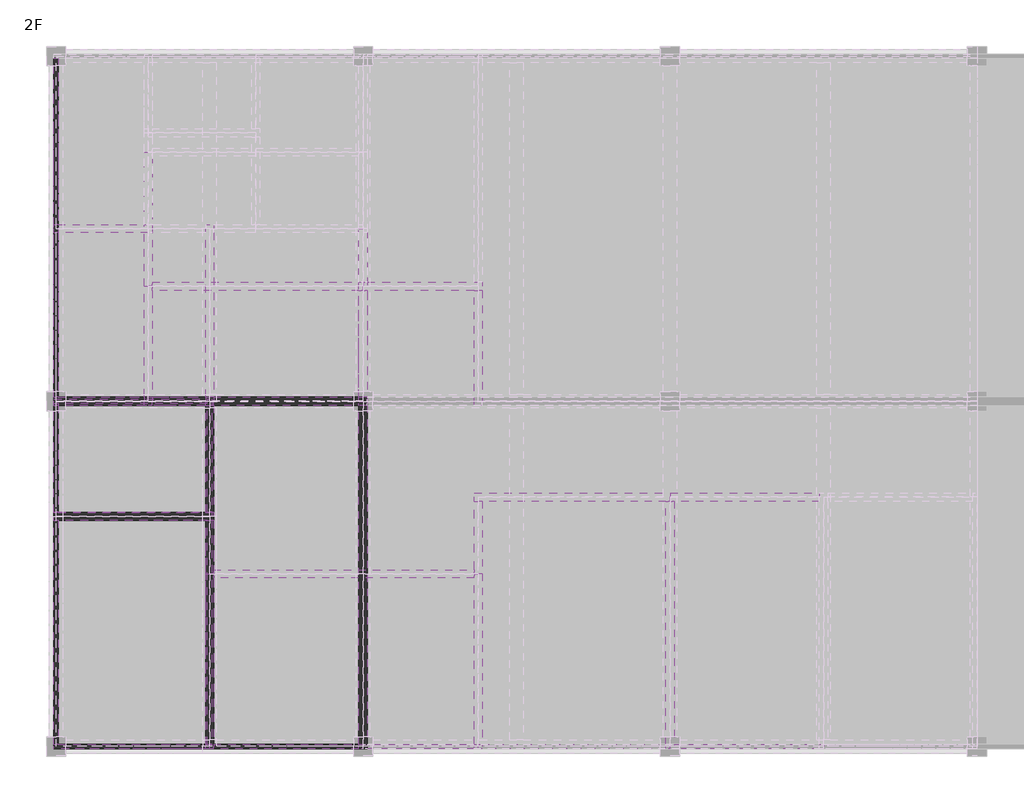
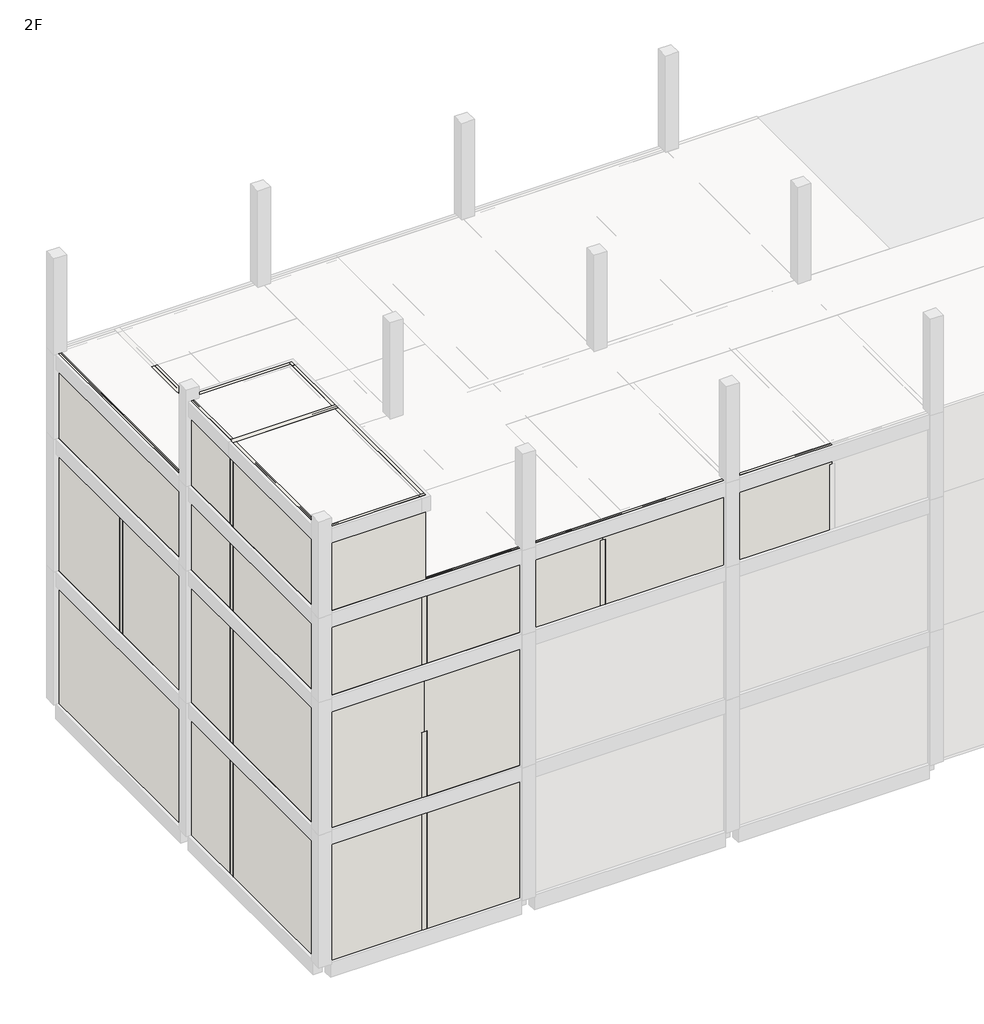
# One storey, part 1 of 7: 58 walls.
"""IFC4 building model written with IfcOpenShell, lengths in millimetres."""

from ifc_helpers import new_model, si_unit, frame, origin, place, context, project, spatial, polyline, outline, extrude, faceted_brep, element, save

model = new_model("IFC4")

# Units and contexts
model_context = context("Model", 3, world=origin())
ifc_project = project(units=[si_unit("LENGTHUNIT", "METRE", prefix="MILLI")], contexts=[model_context])

# Site, building, storey
site = spatial("IfcSite", under=ifc_project)
building = spatial("IfcBuilding", under=site)
storey = spatial("IfcBuildingStorey", under=building, Name="2F", Elevation=3500.0)

# Walls
placement = place(None, origin())
element("IfcWall", 1, ObjectType="WA211_Exterior-Cement Brick-90mm", at=placement, inside=storey, context=model_context, shape_type="SweptSolid", body=[
    extrude(outline(polyline([(45516.6521483, 181866.8614395), (45516.6521483, 173030.8614395), (45402.6521483, 173030.8614395), (45402.6521483, 181866.8614395), (45516.6521483, 181866.8614395)])), frame((0.0, 0.0, 3500.0), z_axis=(0.0, 0.0, 1.0), x_axis=(1.0, 0.0, 0.0)), (0.0, 0.0, 1.0), 5500.0),
])
element("IfcWall", 2, ObjectType="WA211_Exterior-Cement Brick-90mm", at=placement, inside=storey, context=model_context, shape_type="SweptSolid", body=[
    extrude(outline(polyline([(49566.6521483, 163980.8614395), (53352.6521483, 163980.8614395), (53352.6521483, 163866.8614395), (49566.6521483, 163866.8614395), (49566.6521483, 163980.8614395)])), frame((0.0, 0.0, 3500.0), z_axis=(0.0, 0.0, 1.0), x_axis=(1.0, 0.0, 0.0)), (0.0, 0.0, 1.0), 5500.0),
])
element("IfcWall", 3, ObjectType="WA211_Exterior-Cement Brick-90mm", at=placement, inside=storey, context=model_context, shape_type="SweptSolid", body=[
    extrude(outline(polyline([(45516.6521483, 172816.8614395), (45516.6521483, 170030.8614395), (45402.6521483, 170030.8614395), (45402.6521483, 172816.8614395), (45516.6521483, 172816.8614395)])), frame((0.0, 0.0, 3500.0), z_axis=(0.0, 0.0, 1.0), x_axis=(1.0, 0.0, 0.0)), (0.0, 0.0, 1.0), 5500.0),
])
element("IfcWall", 4, ObjectType="WA211_Exterior-Cement Brick-90mm", at=placement, inside=storey, context=model_context, shape_type="SweptSolid", body=[
    extrude(outline(polyline([(45516.6521483, 169816.8614395), (45516.6521483, 163980.8614395), (45402.6521483, 163980.8614395), (45402.6521483, 169816.8614395), (45516.6521483, 169816.8614395)])), frame((0.0, 0.0, 3500.0), z_axis=(0.0, 0.0, 1.0), x_axis=(1.0, 0.0, 0.0)), (0.0, 0.0, 1.0), 5500.0),
])
element("IfcWall", 5, ObjectType="WA211_Exterior-Cement Brick-90mm", at=placement, inside=storey, context=model_context, shape_type="Brep", body=[
    faceted_brep([(49352.6521483, 163980.8614395, 3500.0), (45516.6521483, 163980.8614395, 3500.0), (45402.6521483, 163980.8614395, 3500.0), (45402.6521483, 163980.8614395, 9000.0), (45516.6521483, 163980.8614395, 9000.0), (49352.6521483, 163980.8614395, 9000.0), (49352.6521483, 163866.8614395, 3500.0), (49352.6521483, 163866.8614395, 9000.0), (45402.6521483, 163866.8614395, 9000.0), (45402.6521483, 163866.8614395, 3500.0)], [[[0, 1, 2, 3, 4, 5]], [[6, 7, 8, 9]], [[2, 1, 0, 6, 9]], [[5, 4, 3, 8, 7]], [[0, 5, 7, 6]], [[3, 2, 9, 8]]]),
])
element("IfcWall", 6, ObjectType="WA211_Exterior-Cement Brick-90mm", at=placement, inside=storey, context=model_context, shape_type="SweptSolid", body=[
    extrude(outline(polyline([(45516.6521483, 181866.8614395), (45516.6521483, 177530.8614395), (45402.6521483, 177530.8614395), (45402.6521483, 181866.8614395), (45516.6521483, 181866.8614395)])), frame((0.0, 0.0, 9000.0), z_axis=(0.0, 0.0, 1.0), x_axis=(1.0, 0.0, 0.0)), (0.0, 0.0, 1.0), 5500.0),
])
element("IfcWall", 7, ObjectType="WA211_Exterior-Cement Brick-90mm", at=placement, inside=storey, context=model_context, shape_type="SweptSolid", body=[
    extrude(outline(polyline([(45516.6521483, 177316.8614395), (45516.6521483, 173030.8614395), (45402.6521483, 173030.8614395), (45402.6521483, 177316.8614395), (45516.6521483, 177316.8614395)])), frame((0.0, 0.0, 9000.0), z_axis=(0.0, 0.0, 1.0), x_axis=(1.0, 0.0, 0.0)), (0.0, 0.0, 1.0), 5500.0),
])
element("IfcWall", 8, ObjectType="WA211_Exterior-Cement Brick-90mm", at=placement, inside=storey, context=model_context, shape_type="SweptSolid", body=[
    extrude(outline(polyline([(45516.6521483, 172816.8614395), (45516.6521483, 170030.8614395), (45402.6521483, 170030.8614395), (45402.6521483, 172816.8614395), (45516.6521483, 172816.8614395)])), frame((0.0, 0.0, 9000.0), z_axis=(0.0, 0.0, 1.0), x_axis=(1.0, 0.0, 0.0)), (0.0, 0.0, 1.0), 5500.0),
])
element("IfcWall", 9, ObjectType="WA211_Exterior-Cement Brick-90mm", at=placement, inside=storey, context=model_context, shape_type="SweptSolid", body=[
    extrude(outline(polyline([(45516.6521483, 169816.8614395), (45516.6521483, 163980.8614395), (45402.6521483, 163980.8614395), (45402.6521483, 169816.8614395), (45516.6521483, 169816.8614395)])), frame((0.0, 0.0, 9000.0), z_axis=(0.0, 0.0, 1.0), x_axis=(1.0, 0.0, 0.0)), (0.0, 0.0, 1.0), 5500.0),
])
element("IfcWall", 10, ObjectType="WA211_Exterior-Cement Brick-90mm", at=placement, inside=storey, context=model_context, shape_type="Brep", body=[
    faceted_brep([(49352.6521483, 163980.8614395, 9000.0), (45516.6521483, 163980.8614395, 9000.0), (45402.6521483, 163980.8614395, 9000.0), (45402.6521483, 163980.8614395, 14500.0), (45516.6521483, 163980.8614395, 14500.0), (49459.6521483, 163980.8614395, 14500.0), (49459.6521483, 163980.8614395, 11700.0), (49352.6521483, 163980.8614395, 11700.0), (49352.6521483, 163866.8614395, 9000.0), (49352.6521483, 163866.8614395, 11700.0), (49459.6521483, 163866.8614395, 11700.0), (49459.6521483, 163866.8614395, 14500.0), (45402.6521483, 163866.8614395, 14500.0), (45402.6521483, 163866.8614395, 9000.0)], [[[0, 1, 2, 3, 4, 5, 6, 7]], [[8, 9, 10, 11, 12, 13]], [[2, 1, 0, 8, 13]], [[5, 4, 3, 12, 11]], [[3, 2, 13, 12]], [[6, 5, 11, 10]], [[6, 10, 9, 7]], [[0, 7, 9, 8]]]),
])
element("IfcWall", 11, ObjectType="WA211_Exterior-Cement Brick-90mm", at=placement, inside=storey, context=model_context, shape_type="SweptSolid", body=[
    extrude(outline(polyline([(9000.0, 53352.6521483), (12000.0, 53352.6521483), (12000.0, 53459.6521483), (14500.0, 53459.6521483), (14500.0, 49459.6521483), (11700.0, 49459.6521483), (11700.0, 49566.6521483), (9000.0, 49566.6521483), (9000.0, 53352.6521483)])), frame((0.0, 163866.8614395, 0.0), z_axis=(0.0, 1.0, 0.0), x_axis=(0.0, 0.0, 1.0)), (0.0, 0.0, 1.0), 114.0),
])
element("IfcWall", 12, ObjectType="WA211_Exterior-Cement Brick-90mm", at=placement, inside=storey, context=model_context, shape_type="SweptSolid", body=[
    extrude(outline(polyline([(14500.0, 65352.6521483), (17200.0, 65352.6521483), (17200.0, 65459.6521483), (18000.0, 65459.6521483), (18000.0, 61459.6521483), (17200.0, 61459.6521483), (17200.0, 61566.6521483), (14500.0, 61566.6521483), (14500.0, 65352.6521483)])), frame((0.0, 163866.8614395, 0.0), z_axis=(0.0, 1.0, 0.0), x_axis=(0.0, 0.0, 1.0)), (0.0, 0.0, 1.0), 114.0),
])
element("IfcWall", 13, ObjectType="WA211_Exterior-Cement Brick-90mm", at=placement, inside=storey, context=model_context, shape_type="SweptSolid", body=[
    extrude(outline(polyline([(14500.0, 61352.6521483), (17200.0, 61352.6521483), (17200.0, 61459.6521483), (18000.0, 61459.6521483), (18000.0, 56459.6521483), (17200.0, 56459.6521483), (17200.0, 56566.6521483), (14500.0, 56566.6521483), (14500.0, 61352.6521483)])), frame((0.0, 163866.8614395, 0.0), z_axis=(0.0, 1.0, 0.0), x_axis=(0.0, 0.0, 1.0)), (0.0, 0.0, 1.0), 114.0),
])
element("IfcWall", 14, ObjectType="WA211_Exterior-Cement Brick-90mm", at=placement, inside=storey, context=model_context, shape_type="SweptSolid", body=[
    extrude(outline(polyline([(14500.0, 56352.6521483), (17200.0, 56352.6521483), (17200.0, 56459.6521483), (18000.0, 56459.6521483), (18000.0, 49566.6521483), (14500.0, 49566.6521483), (14500.0, 56352.6521483)])), frame((0.0, 163866.8614395, 0.0), z_axis=(0.0, 1.0, 0.0), x_axis=(0.0, 0.0, 1.0)), (0.0, 0.0, 1.0), 114.0),
])
element("IfcWall", 15, ObjectType="WA211_Exterior-Cement Brick-90mm", at=placement, inside=storey, context=model_context, shape_type="SweptSolid", body=[
    extrude(outline(polyline([(45516.6521483, 181866.8614395), (45516.6521483, 173030.8614395), (45402.6521483, 173030.8614395), (45402.6521483, 181866.8614395), (45516.6521483, 181866.8614395)])), frame((0.0, 0.0, 14500.0), z_axis=(0.0, 0.0, 1.0), x_axis=(1.0, 0.0, 0.0)), (0.0, 0.0, 1.0), 3500.0),
])
element("IfcWall", 16, ObjectType="WA211_Exterior-Cement Brick-90mm", at=placement, inside=storey, context=model_context, shape_type="SweptSolid", body=[
    extrude(outline(polyline([(45516.6521483, 172816.8614395), (45516.6521483, 170030.8614395), (45402.6521483, 170030.8614395), (45402.6521483, 172816.8614395), (45516.6521483, 172816.8614395)])), frame((0.0, 0.0, 14500.0), z_axis=(0.0, 0.0, 1.0), x_axis=(1.0, 0.0, 0.0)), (0.0, 0.0, 1.0), 3500.0),
])
element("IfcWall", 17, ObjectType="WA211_Exterior-Cement Brick-90mm", at=placement, inside=storey, context=model_context, shape_type="SweptSolid", body=[
    extrude(outline(polyline([(45516.6521483, 169816.8614395), (45516.6521483, 163980.8614395), (45402.6521483, 163980.8614395), (45402.6521483, 169816.8614395), (45516.6521483, 169816.8614395)])), frame((0.0, 0.0, 14500.0), z_axis=(0.0, 0.0, 1.0), x_axis=(1.0, 0.0, 0.0)), (0.0, 0.0, 1.0), 3500.0),
])
element("IfcWall", 18, ObjectType="WA211_Exterior-Cement Brick-90mm", at=placement, inside=storey, context=model_context, shape_type="Brep", body=[
    faceted_brep([(49352.6521483, 163980.8614395, 14500.0), (45516.6521483, 163980.8614395, 14500.0), (45402.6521483, 163980.8614395, 14500.0), (45402.6521483, 163980.8614395, 18000.0), (45516.6521483, 163980.8614395, 18000.0), (49352.6521483, 163980.8614395, 18000.0), (49352.6521483, 163866.8614395, 14500.0), (49352.6521483, 163866.8614395, 18000.0), (45402.6521483, 163866.8614395, 18000.0), (45402.6521483, 163866.8614395, 14500.0)], [[[0, 1, 2, 3, 4, 5]], [[6, 7, 8, 9]], [[2, 1, 0, 6, 9]], [[5, 4, 3, 8, 7]], [[0, 5, 7, 6]], [[3, 2, 9, 8]]]),
])
element("IfcWall", 19, ObjectType="WA211_Exterior-Cement Brick-90mm", at=placement, inside=storey, context=model_context, shape_type="Brep", body=[
    faceted_brep([(49402.6521483, 172980.8614395, 18000.0), (49402.6521483, 172866.8614395, 18000.0), (49402.6521483, 170030.8614395, 18000.0), (49402.6521483, 170030.8614395, 21500.0), (49402.6521483, 172866.8614395, 21500.0), (49402.6521483, 172980.8614395, 21500.0), (49516.6521483, 172980.8614395, 18000.0), (49516.6521483, 172980.8614395, 21500.0), (49516.6521483, 170030.8614395, 21500.0), (49516.6521483, 170030.8614395, 18000.0)], [[[0, 1, 2, 3, 4, 5]], [[6, 7, 8, 9]], [[2, 1, 0, 6, 9]], [[5, 4, 3, 8, 7]], [[0, 5, 7, 6]], [[3, 2, 9, 8]]]),
])
element("IfcWall", 20, ObjectType="WA211_Exterior-Cement Brick-90mm", at=placement, inside=storey, context=model_context, shape_type="SweptSolid", body=[
    extrude(outline(polyline([(45516.6521483, 172866.8614395), (45516.6521483, 170030.8614395), (45402.6521483, 170030.8614395), (45402.6521483, 172866.8614395), (45516.6521483, 172866.8614395)])), frame((0.0, 0.0, 18000.0), z_axis=(0.0, 0.0, 1.0), x_axis=(1.0, 0.0, 0.0)), (0.0, 0.0, 1.0), 3500.0),
])
element("IfcWall", 21, ObjectType="WA211_Exterior-Cement Brick-90mm", at=placement, inside=storey, context=model_context, shape_type="Brep", body=[
    faceted_brep([(45402.6521483, 172866.8614395, 18000.0), (45516.6521483, 172866.8614395, 18000.0), (49402.6521483, 172866.8614395, 18000.0), (49402.6521483, 172866.8614395, 21500.0), (45516.6521483, 172866.8614395, 21500.0), (45402.6521483, 172866.8614395, 21500.0), (45402.6521483, 172980.8614395, 18000.0), (45402.6521483, 172980.8614395, 21500.0), (49402.6521483, 172980.8614395, 21500.0), (49402.6521483, 172980.8614395, 18000.0)], [[[0, 1, 2, 3, 4, 5]], [[6, 7, 8, 9]], [[2, 1, 0, 6, 9]], [[5, 4, 3, 8, 7]], [[0, 5, 7, 6]], [[3, 2, 9, 8]]]),
])
element("IfcWall", 22, ObjectType="WA211_Exterior-Cement Brick-90mm", at=placement, inside=storey, context=model_context, shape_type="SweptSolid", body=[
    extrude(outline(polyline([(45516.6521483, 169816.8614395), (45516.6521483, 163980.8614395), (45402.6521483, 163980.8614395), (45402.6521483, 169816.8614395), (45516.6521483, 169816.8614395)])), frame((0.0, 0.0, 18000.0), z_axis=(0.0, 0.0, 1.0), x_axis=(1.0, 0.0, 0.0)), (0.0, 0.0, 1.0), 3500.0),
])
element("IfcWall", 23, ObjectType="WA211_Exterior-Cement Brick-90mm", at=placement, inside=storey, context=model_context, shape_type="Brep", body=[
    faceted_brep([(49516.6521483, 163980.8614395, 18000.0), (49402.6521483, 163980.8614395, 18000.0), (45516.6521483, 163980.8614395, 18000.0), (45402.6521483, 163980.8614395, 18000.0), (45402.6521483, 163980.8614395, 21500.0), (45516.6521483, 163980.8614395, 21500.0), (49402.6521483, 163980.8614395, 21500.0), (49516.6521483, 163980.8614395, 21500.0), (49516.6521483, 163866.8614395, 18000.0), (49516.6521483, 163866.8614395, 21500.0), (45402.6521483, 163866.8614395, 21500.0), (45402.6521483, 163866.8614395, 18000.0)], [[[0, 1, 2, 3, 4, 5, 6, 7]], [[8, 9, 10, 11]], [[3, 2, 1, 0, 8, 11]], [[7, 6, 5, 4, 10, 9]], [[0, 7, 9, 8]], [[4, 3, 11, 10]]]),
])
element("IfcWall", 24, ObjectType="WA211_Exterior-Cement Brick-90mm", at=placement, inside=storey, context=model_context, shape_type="SweptSolid", body=[
    extrude(outline(polyline([(49402.6521483, 163980.8614395), (49402.6521483, 169816.8614395), (49516.6521483, 169816.8614395), (49516.6521483, 163980.8614395), (49402.6521483, 163980.8614395)])), frame((0.0, 0.0, 18000.0), z_axis=(0.0, 0.0, 1.0), x_axis=(1.0, 0.0, 0.0)), (0.0, 0.0, 1.0), 3500.0),
])
element("IfcWall", 25, ObjectType="WA221_Interior-Cement Block-190mm", at=placement, inside=storey, context=model_context, shape_type="SweptSolid", body=[
    extrude(outline(polyline([(49566.6521483, 173030.8614395), (53352.6521483, 173030.8614395), (53352.6521483, 172816.8614395), (49566.6521483, 172816.8614395), (49566.6521483, 173030.8614395)])), frame((0.0, 0.0, 3500.0), z_axis=(0.0, 0.0, 1.0), x_axis=(1.0, 0.0, 0.0)), (0.0, 0.0, 1.0), 5500.0),
])
element("IfcWall", 26, ObjectType="WA221_Interior-Cement Block-190mm", at=placement, inside=storey, context=model_context, shape_type="Brep", body=[
    faceted_brep([(45402.6521483, 172816.8614395, 3500.0), (45516.6521483, 172816.8614395, 3500.0), (49352.6521483, 172816.8614395, 3500.0), (49352.6521483, 172816.8614395, 9000.0), (45516.6521483, 172816.8614395, 9000.0), (45402.6521483, 172816.8614395, 9000.0), (45402.6521483, 173030.8614395, 3500.0), (45402.6521483, 173030.8614395, 9000.0), (45516.6521483, 173030.8614395, 9000.0), (49352.6521483, 173030.8614395, 9000.0), (49352.6521483, 173030.8614395, 3500.0), (45516.6521483, 173030.8614395, 3500.0)], [[[0, 1, 2, 3, 4, 5]], [[6, 7, 8, 9, 10, 11]], [[2, 1, 0, 6, 11, 10]], [[5, 4, 3, 9, 8, 7]], [[0, 5, 7, 6]], [[3, 2, 10, 9]]]),
])
element("IfcWall", 27, ObjectType="WA221_Interior-Cement Block-190mm", at=placement, inside=storey, context=model_context, shape_type="Brep", body=[
    faceted_brep([(53566.6521483, 163866.8614395, 3500.0), (53566.6521483, 163980.8614395, 3500.0), (53566.6521483, 172816.8614395, 3500.0), (53566.6521483, 173030.8614395, 3500.0), (53566.6521483, 173030.8614395, 9000.0), (53566.6521483, 172816.8614395, 9000.0), (53566.6521483, 163980.8614395, 9000.0), (53566.6521483, 163866.8614395, 9000.0), (53352.6521483, 163866.8614395, 3500.0), (53352.6521483, 163866.8614395, 9000.0), (53352.6521483, 163980.8614395, 9000.0), (53352.6521483, 172816.8614395, 9000.0), (53352.6521483, 173030.8614395, 9000.0), (53352.6521483, 173030.8614395, 3500.0), (53352.6521483, 172816.8614395, 3500.0), (53352.6521483, 163980.8614395, 3500.0)], [[[0, 1, 2, 3, 4, 5, 6, 7]], [[8, 9, 10, 11, 12, 13, 14, 15]], [[3, 2, 1, 0, 8, 15, 14, 13]], [[7, 6, 5, 4, 12, 11, 10, 9]], [[0, 7, 9, 8]], [[4, 3, 13, 12]]]),
])
element("IfcWall", 28, ObjectType="WA221_Interior-Cement Block-190mm", at=placement, inside=storey, context=model_context, shape_type="Brep", body=[
    faceted_brep([(49352.6521483, 173030.8614395, 3500.0), (49352.6521483, 172816.8614395, 3500.0), (49352.6521483, 170030.8614395, 3500.0), (49352.6521483, 170030.8614395, 9000.0), (49352.6521483, 172816.8614395, 9000.0), (49352.6521483, 173030.8614395, 9000.0), (49566.6521483, 173030.8614395, 3500.0), (49566.6521483, 173030.8614395, 9000.0), (49566.6521483, 172816.8614395, 9000.0), (49566.6521483, 170030.8614395, 9000.0), (49566.6521483, 170030.8614395, 3500.0), (49566.6521483, 172816.8614395, 3500.0)], [[[0, 1, 2, 3, 4, 5]], [[6, 7, 8, 9, 10, 11]], [[2, 1, 0, 6, 11, 10]], [[5, 4, 3, 9, 8, 7]], [[0, 5, 7, 6]], [[3, 2, 10, 9]]]),
])
element("IfcWall", 29, ObjectType="WA221_Interior-Cement Block-190mm", at=placement, inside=storey, context=model_context, shape_type="Brep", body=[
    faceted_brep([(49352.6521483, 169816.8614395, 3500.0), (49352.6521483, 163980.8614395, 3500.0), (49352.6521483, 163866.8614395, 3500.0), (49352.6521483, 163866.8614395, 9000.0), (49352.6521483, 163980.8614395, 9000.0), (49352.6521483, 169816.8614395, 9000.0), (49566.6521483, 169816.8614395, 3500.0), (49566.6521483, 169816.8614395, 9000.0), (49566.6521483, 163980.8614395, 9000.0), (49566.6521483, 163866.8614395, 9000.0), (49566.6521483, 163866.8614395, 3500.0), (49566.6521483, 163980.8614395, 3500.0)], [[[0, 1, 2, 3, 4, 5]], [[6, 7, 8, 9, 10, 11]], [[2, 1, 0, 6, 11, 10]], [[5, 4, 3, 9, 8, 7]], [[3, 2, 10, 9]], [[0, 5, 7, 6]]]),
])
element("IfcWall", 30, ObjectType="WA221_Interior-Cement Block-190mm", at=placement, inside=storey, context=model_context, shape_type="Brep", body=[
    faceted_brep([(45402.6521483, 169816.8614395, 3500.0), (45516.6521483, 169816.8614395, 3500.0), (49352.6521483, 169816.8614395, 3500.0), (49566.6521483, 169816.8614395, 3500.0), (49566.6521483, 169816.8614395, 9000.0), (49352.6521483, 169816.8614395, 9000.0), (45516.6521483, 169816.8614395, 9000.0), (45402.6521483, 169816.8614395, 9000.0), (45402.6521483, 170030.8614395, 3500.0), (45402.6521483, 170030.8614395, 9000.0), (45516.6521483, 170030.8614395, 9000.0), (49352.6521483, 170030.8614395, 9000.0), (49566.6521483, 170030.8614395, 9000.0), (49566.6521483, 170030.8614395, 3500.0), (49352.6521483, 170030.8614395, 3500.0), (45516.6521483, 170030.8614395, 3500.0)], [[[0, 1, 2, 3, 4, 5, 6, 7]], [[8, 9, 10, 11, 12, 13, 14, 15]], [[3, 2, 1, 0, 8, 15, 14, 13]], [[7, 6, 5, 4, 12, 11, 10, 9]], [[0, 7, 9, 8]], [[4, 3, 13, 12]]]),
])
element("IfcWall", 31, ObjectType="WA221_Interior-Cement Block-190mm", at=placement, inside=storey, context=model_context, shape_type="Brep", body=[
    faceted_brep([(53566.6521483, 172923.8614395, 9000.0), (53566.6521483, 173030.8614395, 9000.0), (53566.6521483, 177316.8614395, 9000.0), (53566.6521483, 177316.8614395, 11700.0), (53566.6521483, 177423.8614395, 11700.0), (53566.6521483, 177423.8614395, 12400.0), (53566.6521483, 173030.8614395, 12400.0), (53566.6521483, 172816.8614395, 12400.0), (53566.6521483, 172816.8614395, 12000.0), (53566.6521483, 172923.8614395, 12000.0), (53352.6521483, 172923.8614395, 9000.0), (53352.6521483, 172923.8614395, 12000.0), (53352.6521483, 172816.8614395, 12000.0), (53352.6521483, 172816.8614395, 12400.0), (53352.6521483, 177423.8614395, 12400.0), (53352.6521483, 177423.8614395, 11700.0), (53352.6521483, 177316.8614395, 11700.0), (53352.6521483, 177316.8614395, 9000.0)], [[[0, 1, 2, 3, 4, 5, 6, 7, 8, 9]], [[10, 11, 12, 13, 14, 15, 16, 17]], [[2, 1, 0, 10, 17]], [[7, 6, 5, 14, 13]], [[0, 9, 11, 10]], [[8, 12, 11, 9]], [[8, 7, 13, 12]], [[5, 4, 15, 14]], [[15, 4, 3, 16]], [[3, 2, 17, 16]]]),
])
element("IfcWall", 32, ObjectType="WA221_Interior-Cement Block-190mm", at=placement, inside=storey, context=model_context, shape_type="Brep", body=[
    faceted_brep([(53566.6521483, 163866.8614395, 9000.0), (53566.6521483, 163980.8614395, 9000.0), (53566.6521483, 172816.8614395, 9000.0), (53566.6521483, 172923.8614395, 9000.0), (53566.6521483, 172923.8614395, 12000.0), (53566.6521483, 172816.8614395, 12000.0), (53566.6521483, 163980.8614395, 12000.0), (53566.6521483, 163866.8614395, 12000.0), (53352.6521483, 163866.8614395, 9000.0), (53352.6521483, 163866.8614395, 12000.0), (53352.6521483, 163980.8614395, 12000.0), (53352.6521483, 172816.8614395, 12000.0), (53352.6521483, 172923.8614395, 12000.0), (53352.6521483, 172923.8614395, 9000.0), (53352.6521483, 163980.8614395, 9000.0), (53459.6521483, 163866.8614395, 12000.0)], [[[0, 1, 2, 3, 4, 5, 6, 7]], [[8, 9, 10, 11, 12, 13, 14]], [[3, 2, 1, 0, 8, 14, 13]], [[4, 3, 13, 12]], [[7, 6, 5, 4, 12, 11, 10, 9, 15]], [[0, 7, 15, 9, 8]]]),
])
element("IfcWall", 33, ObjectType="WA221_Interior-Cement Block-190mm", at=placement, inside=storey, context=model_context, shape_type="Brep", body=[
    faceted_brep([(47859.6521483, 177530.8614395, 9000.0), (47752.6521483, 177530.8614395, 9000.0), (45516.6521483, 177530.8614395, 9000.0), (45402.6521483, 177530.8614395, 9000.0), (45402.6521483, 177530.8614395, 14500.0), (45516.6521483, 177530.8614395, 14500.0), (47752.6521483, 177530.8614395, 14500.0), (47966.6521483, 177530.8614395, 14500.0), (47966.6521483, 177530.8614395, 11700.0), (47859.6521483, 177530.8614395, 11700.0), (47859.6521483, 177316.8614395, 9000.0), (47859.6521483, 177316.8614395, 11700.0), (47966.6521483, 177316.8614395, 11700.0), (47966.6521483, 177316.8614395, 14500.0), (45516.6521483, 177316.8614395, 14500.0), (45402.6521483, 177316.8614395, 14500.0), (45402.6521483, 177316.8614395, 9000.0), (45516.6521483, 177316.8614395, 9000.0)], [[[0, 1, 2, 3, 4, 5, 6, 7, 8, 9]], [[10, 11, 12, 13, 14, 15, 16, 17]], [[3, 2, 1, 0, 10, 17, 16]], [[7, 6, 5, 4, 15, 14, 13]], [[0, 9, 11, 10]], [[8, 12, 11, 9]], [[8, 7, 13, 12]], [[4, 3, 16, 15]]]),
])
element("IfcWall", 34, ObjectType="WA221_Interior-Cement Block-190mm", at=placement, inside=storey, context=model_context, shape_type="Brep", body=[
    faceted_brep([(45402.6521483, 172816.8614395, 9000.0), (45516.6521483, 172816.8614395, 9000.0), (49352.6521483, 172816.8614395, 9000.0), (49566.6521483, 172816.8614395, 9000.0), (49566.6521483, 172816.8614395, 14500.0), (49352.6521483, 172816.8614395, 14500.0), (45516.6521483, 172816.8614395, 14500.0), (45402.6521483, 172816.8614395, 14500.0), (45402.6521483, 173030.8614395, 9000.0), (45402.6521483, 173030.8614395, 14500.0), (45516.6521483, 173030.8614395, 14500.0), (49566.6521483, 173030.8614395, 14500.0), (49566.6521483, 173030.8614395, 11700.0), (49566.6521483, 173030.8614395, 9000.0), (49352.6521483, 173030.8614395, 9000.0), (45516.6521483, 173030.8614395, 9000.0)], [[[0, 1, 2, 3, 4, 5, 6, 7]], [[8, 9, 10, 11, 12, 13, 14, 15]], [[3, 2, 1, 0, 8, 15, 14, 13]], [[7, 6, 5, 4, 11, 10, 9]], [[0, 7, 9, 8]], [[3, 13, 12, 11, 4]]]),
])
element("IfcWall", 35, ObjectType="WA221_Interior-Cement Block-190mm", at=placement, inside=storey, context=model_context, shape_type="Brep", body=[
    faceted_brep([(49352.6521483, 177530.8614395, 9000.0), (49352.6521483, 177316.8614395, 9000.0), (49352.6521483, 173030.8614395, 9000.0), (49352.6521483, 173030.8614395, 11700.0), (49352.6521483, 177316.8614395, 11700.0), (49352.6521483, 177530.8614395, 11700.0), (49566.6521483, 177530.8614395, 9000.0), (49566.6521483, 177530.8614395, 11700.0), (49566.6521483, 177316.8614395, 11700.0), (49566.6521483, 173030.8614395, 11700.0), (49566.6521483, 173030.8614395, 9000.0), (49566.6521483, 177316.8614395, 9000.0)], [[[0, 1, 2, 3, 4, 5]], [[6, 7, 8, 9, 10, 11]], [[2, 1, 0, 6, 11, 10]], [[5, 4, 3, 9, 8, 7]], [[0, 5, 7, 6]], [[3, 2, 10, 9]]]),
])
element("IfcWall", 36, ObjectType="WA221_Interior-Cement Block-190mm", at=placement, inside=storey, context=model_context, shape_type="Brep", body=[
    faceted_brep([(49566.6521483, 170030.8614395, 14500.0), (49566.6521483, 170030.8614395, 9000.0), (49352.6521483, 170030.8614395, 9000.0), (45516.6521483, 170030.8614395, 9000.0), (45402.6521483, 170030.8614395, 9000.0), (45402.6521483, 170030.8614395, 14500.0), (45516.6521483, 170030.8614395, 14500.0), (49352.6521483, 170030.8614395, 14500.0), (49566.6521483, 169816.8614395, 9000.0), (49566.6521483, 169816.8614395, 11700.0), (49566.6521483, 169816.8614395, 14500.0), (45516.6521483, 169816.8614395, 14500.0), (45402.6521483, 169816.8614395, 14500.0), (45402.6521483, 169816.8614395, 9000.0), (45516.6521483, 169816.8614395, 9000.0), (49352.6521483, 169816.8614395, 9000.0)], [[[0, 1, 2, 3, 4, 5, 6, 7]], [[8, 9, 10, 11, 12, 13, 14, 15]], [[4, 3, 2, 1, 8, 15, 14, 13]], [[0, 7, 6, 5, 12, 11, 10]], [[5, 4, 13, 12]], [[0, 10, 9, 8, 1]]]),
])
element("IfcWall", 37, ObjectType="WA221_Interior-Cement Block-190mm", at=placement, inside=storey, context=model_context, shape_type="SweptSolid", body=[
    extrude(outline(polyline([(49352.6521483, 170030.8614395), (49352.6521483, 172816.8614395), (49566.6521483, 172816.8614395), (49566.6521483, 170030.8614395), (49352.6521483, 170030.8614395)])), frame((0.0, 0.0, 9000.0), z_axis=(0.0, 0.0, 1.0), x_axis=(1.0, 0.0, 0.0)), (0.0, 0.0, 1.0), 5500.0),
])
element("IfcWall", 38, ObjectType="WA221_Interior-Cement Block-190mm", at=placement, inside=storey, context=model_context, shape_type="Brep", body=[
    faceted_brep([(49352.6521483, 169816.8614395, 9000.0), (49352.6521483, 163980.8614395, 9000.0), (49352.6521483, 163866.8614395, 9000.0), (49352.6521483, 163866.8614395, 11700.0), (49352.6521483, 163980.8614395, 11700.0), (49352.6521483, 169816.8614395, 11700.0), (49566.6521483, 169816.8614395, 9000.0), (49566.6521483, 169816.8614395, 11700.0), (49566.6521483, 163980.8614395, 11700.0), (49566.6521483, 163866.8614395, 11700.0), (49566.6521483, 163866.8614395, 9000.0), (49566.6521483, 163980.8614395, 9000.0), (49459.6521483, 163866.8614395, 11700.0)], [[[0, 1, 2, 3, 4, 5]], [[6, 7, 8, 9, 10, 11]], [[2, 1, 0, 6, 11, 10]], [[5, 4, 3, 12, 9, 8, 7]], [[0, 5, 7, 6]], [[3, 2, 10, 9, 12]]]),
])
element("IfcWall", 39, ObjectType="WA221_Interior-Cement Block-190mm", at=placement, inside=storey, context=model_context, shape_type="Brep", body=[
    faceted_brep([(61352.6521483, 170316.8614395, 14500.0), (61352.6521483, 163980.8614395, 14500.0), (61352.6521483, 163866.8614395, 14500.0), (61352.6521483, 163866.8614395, 17200.0), (61352.6521483, 163980.8614395, 17200.0), (61352.6521483, 170316.8614395, 17200.0), (61566.6521483, 170316.8614395, 14500.0), (61566.6521483, 170316.8614395, 17200.0), (61566.6521483, 163980.8614395, 17200.0), (61566.6521483, 163866.8614395, 17200.0), (61566.6521483, 163866.8614395, 14500.0), (61566.6521483, 163980.8614395, 14500.0), (61459.6521483, 170316.8614395, 14500.0), (61459.6521483, 163866.8614395, 17200.0), (61459.6521483, 170316.8614395, 17200.0)], [[[0, 1, 2, 3, 4, 5]], [[6, 7, 8, 9, 10, 11]], [[2, 1, 0, 12, 6, 11, 10]], [[5, 4, 3, 13, 9, 8, 7, 14]], [[3, 2, 10, 9, 13]], [[0, 5, 14, 7, 6, 12]]]),
])
element("IfcWall", 40, ObjectType="WA221_Interior-Cement Block-190mm", at=placement, inside=storey, context=model_context, shape_type="Brep", body=[
    faceted_brep([(61459.6521483, 170316.8614395, 14500.0), (61566.6521483, 170316.8614395, 14500.0), (65352.6521483, 170316.8614395, 14500.0), (65352.6521483, 170316.8614395, 17200.0), (61566.6521483, 170316.8614395, 17200.0), (61459.6521483, 170316.8614395, 17200.0), (61459.6521483, 170530.8614395, 14500.0), (61459.6521483, 170530.8614395, 17200.0), (65352.6521483, 170530.8614395, 17200.0), (65352.6521483, 170530.8614395, 14500.0)], [[[0, 1, 2, 3, 4, 5]], [[6, 7, 8, 9]], [[2, 1, 0, 6, 9]], [[5, 4, 3, 8, 7]], [[0, 5, 7, 6]], [[3, 2, 9, 8]]]),
])
element("IfcWall", 41, ObjectType="WA221_Interior-Cement Block-190mm", at=placement, inside=storey, context=model_context, shape_type="Brep", body=[
    faceted_brep([(56566.6521483, 172816.8614395, 14500.0), (56566.6521483, 173030.8614395, 14500.0), (56566.6521483, 175816.8614395, 14500.0), (56566.6521483, 175816.8614395, 17200.0), (56566.6521483, 173030.8614395, 17200.0), (56566.6521483, 172816.8614395, 17200.0), (56352.6521483, 172816.8614395, 14500.0), (56352.6521483, 172816.8614395, 17200.0), (56352.6521483, 175816.8614395, 17200.0), (56352.6521483, 175816.8614395, 14500.0)], [[[0, 1, 2, 3, 4, 5]], [[6, 7, 8, 9]], [[2, 1, 0, 6, 9]], [[5, 4, 3, 8, 7]], [[0, 5, 7, 6]], [[3, 2, 9, 8]]]),
])
element("IfcWall", 42, ObjectType="WA221_Interior-Cement Block-190mm", at=placement, inside=storey, context=model_context, shape_type="Brep", body=[
    faceted_brep([(56566.6521483, 163866.8614395, 14500.0), (56566.6521483, 163980.8614395, 14500.0), (56566.6521483, 168423.8614395, 14500.0), (56566.6521483, 168423.8614395, 17200.0), (56566.6521483, 163980.8614395, 17200.0), (56566.6521483, 163866.8614395, 17200.0), (56352.6521483, 163866.8614395, 14500.0), (56352.6521483, 163866.8614395, 17200.0), (56352.6521483, 163980.8614395, 17200.0), (56352.6521483, 168316.8614395, 17200.0), (56352.6521483, 168423.8614395, 17200.0), (56352.6521483, 168423.8614395, 14500.0), (56352.6521483, 168316.8614395, 14500.0), (56352.6521483, 163980.8614395, 14500.0), (56459.6521483, 163866.8614395, 17200.0)], [[[0, 1, 2, 3, 4, 5]], [[6, 7, 8, 9, 10, 11, 12, 13]], [[2, 1, 0, 6, 13, 12, 11]], [[3, 2, 11, 10]], [[5, 4, 3, 10, 9, 8, 7, 14]], [[0, 5, 14, 7, 6]]]),
])
element("IfcWall", 43, ObjectType="WA221_Interior-Cement Block-190mm", at=placement, inside=storey, context=model_context, shape_type="Brep", body=[
    faceted_brep([(56352.6521483, 170316.8614395, 14500.0), (56566.6521483, 170316.8614395, 14500.0), (61352.6521483, 170316.8614395, 14500.0), (61459.6521483, 170316.8614395, 14500.0), (61459.6521483, 170316.8614395, 17200.0), (61352.6521483, 170316.8614395, 17200.0), (56566.6521483, 170316.8614395, 17200.0), (56352.6521483, 170316.8614395, 17200.0), (56352.6521483, 170530.8614395, 14500.0), (56352.6521483, 170530.8614395, 17200.0), (61459.6521483, 170530.8614395, 17200.0), (61459.6521483, 170530.8614395, 14500.0)], [[[0, 1, 2, 3, 4, 5, 6, 7]], [[8, 9, 10, 11]], [[3, 2, 1, 0, 8, 11]], [[4, 3, 11, 10]], [[7, 6, 5, 4, 10, 9]], [[0, 7, 9, 8]]]),
])
element("IfcWall", 44, ObjectType="WA221_Interior-Cement Block-190mm", at=placement, inside=storey, context=model_context, shape_type="Brep", body=[
    faceted_brep([(56566.6521483, 168423.8614395, 14500.0), (56566.6521483, 170316.8614395, 14500.0), (56566.6521483, 170316.8614395, 17200.0), (56566.6521483, 168423.8614395, 17200.0), (56352.6521483, 168423.8614395, 14500.0), (56352.6521483, 168423.8614395, 17200.0), (56352.6521483, 168530.8614395, 17200.0), (56352.6521483, 170316.8614395, 17200.0), (56352.6521483, 170316.8614395, 14500.0), (56352.6521483, 168530.8614395, 14500.0)], [[[0, 1, 2, 3]], [[4, 5, 6, 7, 8, 9]], [[1, 0, 4, 9, 8]], [[3, 2, 7, 6, 5]], [[0, 3, 5, 4]], [[2, 1, 8, 7]]]),
])
element("IfcWall", 45, ObjectType="WA221_Interior-Cement Block-190mm", at=placement, inside=storey, context=model_context, shape_type="Brep", body=[
    faceted_brep([(49352.6521483, 168423.8614395, 18000.0), (49352.6521483, 168423.8614395, 14500.0), (49352.6521483, 163980.8614395, 14500.0), (49352.6521483, 163866.8614395, 14500.0), (49352.6521483, 163866.8614395, 18000.0), (49352.6521483, 163980.8614395, 18000.0), (49566.6521483, 168423.8614395, 14500.0), (49566.6521483, 168423.8614395, 18000.0), (49566.6521483, 163980.8614395, 18000.0), (49566.6521483, 163866.8614395, 18000.0), (49566.6521483, 163866.8614395, 14500.0), (49566.6521483, 163980.8614395, 14500.0), (49566.6521483, 168316.8614395, 14500.0)], [[[0, 1, 2, 3, 4, 5]], [[6, 7, 8, 9, 10, 11, 12]], [[3, 2, 1, 6, 12, 11, 10]], [[0, 5, 4, 9, 8, 7]], [[0, 7, 6, 1]], [[4, 3, 10, 9]]]),
])
element("IfcWall", 46, ObjectType="WA221_Interior-Cement Block-190mm", at=placement, inside=storey, context=model_context, shape_type="Brep", body=[
    faceted_brep([(56352.6521483, 168530.8614395, 14500.0), (49566.6521483, 168530.8614395, 14500.0), (49566.6521483, 168530.8614395, 17200.0), (56352.6521483, 168530.8614395, 17200.0), (56352.6521483, 168316.8614395, 14500.0), (56352.6521483, 168316.8614395, 17200.0), (49566.6521483, 168316.8614395, 17200.0), (49566.6521483, 168316.8614395, 14500.0), (56352.6521483, 168423.8614395, 14500.0), (49566.6521483, 168423.8614395, 14500.0), (56352.6521483, 168423.8614395, 17200.0)], [[[0, 1, 2, 3]], [[4, 5, 6, 7]], [[1, 0, 8, 4, 7, 9]], [[3, 2, 6, 5, 10]], [[0, 3, 10, 5, 4, 8]], [[2, 1, 9, 7, 6]]]),
])
element("IfcWall", 47, ObjectType="WA221_Interior-Cement Block-190mm", at=placement, inside=storey, context=model_context, shape_type="Brep", body=[
    faceted_brep([(47966.6521483, 175816.8614395, 14500.0), (53352.6521483, 175816.8614395, 14500.0), (53459.6521483, 175816.8614395, 14500.0), (53459.6521483, 175816.8614395, 17200.0), (53352.6521483, 175816.8614395, 17200.0), (47966.6521483, 175816.8614395, 17200.0), (47966.6521483, 176030.8614395, 14500.0), (47966.6521483, 176030.8614395, 17200.0), (53352.6521483, 176030.8614395, 17200.0), (53459.6521483, 176030.8614395, 17200.0), (53459.6521483, 176030.8614395, 14500.0), (53352.6521483, 176030.8614395, 14500.0), (47966.6521483, 175923.8614395, 14500.0)], [[[0, 1, 2, 3, 4, 5]], [[6, 7, 8, 9, 10, 11]], [[2, 1, 0, 12, 6, 11, 10]], [[3, 2, 10, 9]], [[5, 4, 3, 9, 8, 7]], [[0, 5, 7, 6, 12]]]),
])
element("IfcWall", 48, ObjectType="WA221_Interior-Cement Block-190mm", at=placement, inside=storey, context=model_context, shape_type="Brep", body=[
    faceted_brep([(47752.6521483, 179423.8614395, 18000.0), (47752.6521483, 179423.8614395, 14500.0), (47752.6521483, 175923.8614395, 14500.0), (47752.6521483, 175923.8614395, 18000.0), (47966.6521483, 179423.8614395, 14500.0), (47966.6521483, 179423.8614395, 18000.0), (47966.6521483, 175923.8614395, 18000.0), (47966.6521483, 175923.8614395, 14500.0), (47966.6521483, 176030.8614395, 14500.0), (47966.6521483, 179316.8614395, 14500.0)], [[[0, 1, 2, 3]], [[4, 5, 6, 7, 8, 9]], [[2, 1, 4, 9, 8, 7]], [[0, 3, 6, 5]], [[0, 5, 4, 1]], [[2, 7, 6, 3]]]),
])
element("IfcWall", 49, ObjectType="WA221_Interior-Cement Block-190mm", at=placement, inside=storey, context=model_context, shape_type="Brep", body=[
    faceted_brep([(53459.6521483, 175816.8614395, 14500.0), (53566.6521483, 175816.8614395, 14500.0), (56352.6521483, 175816.8614395, 14500.0), (56566.6521483, 175816.8614395, 14500.0), (56566.6521483, 175816.8614395, 17200.0), (56352.6521483, 175816.8614395, 17200.0), (53566.6521483, 175816.8614395, 17200.0), (53459.6521483, 175816.8614395, 17200.0), (53459.6521483, 176030.8614395, 14500.0), (53459.6521483, 176030.8614395, 17200.0), (53566.6521483, 176030.8614395, 17200.0), (56352.6521483, 176030.8614395, 17200.0), (56566.6521483, 176030.8614395, 17200.0), (56566.6521483, 176030.8614395, 14500.0), (56352.6521483, 176030.8614395, 14500.0), (53566.6521483, 176030.8614395, 14500.0)], [[[0, 1, 2, 3, 4, 5, 6, 7]], [[8, 9, 10, 11, 12, 13, 14, 15]], [[3, 2, 1, 0, 8, 15, 14, 13]], [[7, 6, 5, 4, 12, 11, 10, 9]], [[0, 7, 9, 8]], [[4, 3, 13, 12]]]),
])
element("IfcWall", 50, ObjectType="WA221_Interior-Cement Block-190mm", at=placement, inside=storey, context=model_context, shape_type="Brep", body=[
    faceted_brep([(47752.6521483, 175923.8614395, 18000.0), (47752.6521483, 175923.8614395, 14500.0), (47752.6521483, 173030.8614395, 14500.0), (47752.6521483, 172816.8614395, 14500.0), (47752.6521483, 172816.8614395, 18000.0), (47752.6521483, 173030.8614395, 18000.0), (47966.6521483, 175923.8614395, 14500.0), (47966.6521483, 175923.8614395, 18000.0), (47966.6521483, 173030.8614395, 18000.0), (47966.6521483, 172816.8614395, 18000.0), (47966.6521483, 172816.8614395, 14500.0), (47966.6521483, 173030.8614395, 14500.0), (47966.6521483, 175816.8614395, 14500.0)], [[[0, 1, 2, 3, 4, 5]], [[6, 7, 8, 9, 10, 11, 12]], [[3, 2, 1, 6, 12, 11, 10]], [[0, 5, 4, 9, 8, 7]], [[0, 7, 6, 1]], [[4, 3, 10, 9]]]),
])
element("IfcWall", 51, ObjectType="WA221_Interior-Cement Block-190mm", at=placement, inside=storey, context=model_context, shape_type="SweptSolid", body=[
    extrude(outline(polyline([(49352.6521483, 172816.8614395), (47966.6521483, 172816.8614395), (47966.6521483, 173030.8614395), (49352.6521483, 173030.8614395), (49352.6521483, 172816.8614395)])), frame((0.0, 0.0, 14500.0), z_axis=(0.0, 0.0, 1.0), x_axis=(1.0, 0.0, 0.0)), (0.0, 0.0, 1.0), 3500.0),
])
element("IfcWall", 52, ObjectType="WA221_Interior-Cement Block-190mm", at=placement, inside=storey, context=model_context, shape_type="Brep", body=[
    faceted_brep([(53566.6521483, 173030.8614395, 14500.0), (53352.6521483, 173030.8614395, 14500.0), (49566.6521483, 173030.8614395, 14500.0), (49566.6521483, 173030.8614395, 17200.0), (53352.6521483, 173030.8614395, 17200.0), (53566.6521483, 173030.8614395, 17200.0), (53566.6521483, 172816.8614395, 14500.0), (53566.6521483, 172816.8614395, 17200.0), (49566.6521483, 172816.8614395, 17200.0), (49566.6521483, 172816.8614395, 14500.0)], [[[0, 1, 2, 3, 4, 5]], [[6, 7, 8, 9]], [[2, 1, 0, 6, 9]], [[5, 4, 3, 8, 7]], [[0, 5, 7, 6]], [[3, 2, 9, 8]]]),
])
element("IfcWall", 53, ObjectType="WA221_Interior-Cement Block-190mm", at=placement, inside=storey, context=model_context, shape_type="Brep", body=[
    faceted_brep([(53352.6521483, 175816.8614395, 14500.0), (53352.6521483, 173030.8614395, 14500.0), (53352.6521483, 173030.8614395, 17200.0), (53352.6521483, 175816.8614395, 17200.0), (53566.6521483, 175816.8614395, 14500.0), (53566.6521483, 175816.8614395, 17200.0), (53566.6521483, 173030.8614395, 17200.0), (53566.6521483, 173030.8614395, 14500.0), (53459.6521483, 175816.8614395, 14500.0), (53459.6521483, 175816.8614395, 17200.0)], [[[0, 1, 2, 3]], [[4, 5, 6, 7]], [[1, 0, 8, 4, 7]], [[3, 2, 6, 5, 9]], [[0, 3, 9, 5, 4, 8]], [[2, 1, 7, 6]]]),
])
element("IfcWall", 54, ObjectType="WA221_Interior-Cement Block-190mm", at=placement, inside=storey, context=model_context, shape_type="Brep", body=[
    faceted_brep([(47752.6521483, 173030.8614395, 14500.0), (45516.6521483, 173030.8614395, 14500.0), (45402.6521483, 173030.8614395, 14500.0), (45402.6521483, 173030.8614395, 18000.0), (45516.6521483, 173030.8614395, 18000.0), (47752.6521483, 173030.8614395, 18000.0), (47752.6521483, 172816.8614395, 14500.0), (47752.6521483, 172816.8614395, 18000.0), (45516.6521483, 172816.8614395, 18000.0), (45402.6521483, 172816.8614395, 18000.0), (45402.6521483, 172816.8614395, 14500.0), (45516.6521483, 172816.8614395, 14500.0)], [[[0, 1, 2, 3, 4, 5]], [[6, 7, 8, 9, 10, 11]], [[2, 1, 0, 6, 11, 10]], [[5, 4, 3, 9, 8, 7]], [[0, 5, 7, 6]], [[3, 2, 10, 9]]]),
])
element("IfcWall", 55, ObjectType="WA221_Interior-Cement Block-190mm", at=placement, inside=storey, context=model_context, shape_type="Brep", body=[
    faceted_brep([(45402.6521483, 169816.8614395, 14500.0), (45516.6521483, 169816.8614395, 14500.0), (49352.6521483, 169816.8614395, 14500.0), (49566.6521483, 169816.8614395, 14500.0), (49566.6521483, 169816.8614395, 18000.0), (49352.6521483, 169816.8614395, 18000.0), (45516.6521483, 169816.8614395, 18000.0), (45402.6521483, 169816.8614395, 18000.0), (45402.6521483, 170030.8614395, 14500.0), (45402.6521483, 170030.8614395, 18000.0), (45516.6521483, 170030.8614395, 18000.0), (49352.6521483, 170030.8614395, 18000.0), (49566.6521483, 170030.8614395, 18000.0), (49566.6521483, 170030.8614395, 14500.0), (49352.6521483, 170030.8614395, 14500.0), (45516.6521483, 170030.8614395, 14500.0)], [[[0, 1, 2, 3, 4, 5, 6, 7]], [[8, 9, 10, 11, 12, 13, 14, 15]], [[3, 2, 1, 0, 8, 15, 14, 13]], [[7, 6, 5, 4, 12, 11, 10, 9]], [[0, 7, 9, 8]], [[4, 3, 13, 12]]]),
])
element("IfcWall", 56, ObjectType="WA221_Interior-Cement Block-190mm", at=placement, inside=storey, context=model_context, shape_type="Brep", body=[
    faceted_brep([(49352.6521483, 173030.8614395, 18000.0), (49352.6521483, 173030.8614395, 14500.0), (49352.6521483, 172816.8614395, 14500.0), (49352.6521483, 170030.8614395, 14500.0), (49352.6521483, 170030.8614395, 18000.0), (49352.6521483, 172816.8614395, 18000.0), (49566.6521483, 173030.8614395, 14500.0), (49566.6521483, 173030.8614395, 17200.0), (49566.6521483, 173030.8614395, 18000.0), (49566.6521483, 170030.8614395, 18000.0), (49566.6521483, 170030.8614395, 14500.0), (49566.6521483, 172816.8614395, 14500.0)], [[[0, 1, 2, 3, 4, 5]], [[6, 7, 8, 9, 10, 11]], [[3, 2, 1, 6, 11, 10]], [[0, 5, 4, 9, 8]], [[4, 3, 10, 9]], [[0, 8, 7, 6, 1]]]),
])
element("IfcWall", 57, ObjectType="WA221_Interior-Cement Block-190mm", at=placement, inside=storey, context=model_context, shape_type="Brep", body=[
    faceted_brep([(49352.6521483, 169816.8614395, 14500.0), (49352.6521483, 168423.8614395, 14500.0), (49352.6521483, 168423.8614395, 18000.0), (49352.6521483, 169816.8614395, 18000.0), (49566.6521483, 169816.8614395, 14500.0), (49566.6521483, 169816.8614395, 18000.0), (49566.6521483, 168423.8614395, 18000.0), (49566.6521483, 168423.8614395, 14500.0), (49566.6521483, 168530.8614395, 14500.0)], [[[0, 1, 2, 3]], [[4, 5, 6, 7, 8]], [[1, 0, 4, 8, 7]], [[3, 2, 6, 5]], [[1, 7, 6, 2]], [[0, 3, 5, 4]]]),
])
element("IfcWall", 58, ObjectType="WA221_Interior-Cement Block-190mm", at=placement, inside=storey, context=model_context, shape_type="Brep", body=[
    faceted_brep([(49516.6521483, 170030.8614395, 18000.0), (49402.6521483, 170030.8614395, 18000.0), (45516.6521483, 170030.8614395, 18000.0), (45402.6521483, 170030.8614395, 18000.0), (45402.6521483, 170030.8614395, 21500.0), (45516.6521483, 170030.8614395, 21500.0), (49402.6521483, 170030.8614395, 21500.0), (49516.6521483, 170030.8614395, 21500.0), (49516.6521483, 169816.8614395, 18000.0), (49516.6521483, 169816.8614395, 21500.0), (49402.6521483, 169816.8614395, 21500.0), (45516.6521483, 169816.8614395, 21500.0), (45402.6521483, 169816.8614395, 21500.0), (45402.6521483, 169816.8614395, 18000.0), (45516.6521483, 169816.8614395, 18000.0), (49402.6521483, 169816.8614395, 18000.0)], [[[0, 1, 2, 3, 4, 5, 6, 7]], [[8, 9, 10, 11, 12, 13, 14, 15]], [[3, 2, 1, 0, 8, 15, 14, 13]], [[7, 6, 5, 4, 12, 11, 10, 9]], [[4, 3, 13, 12]], [[0, 7, 9, 8]]]),
])

save(model, "model.ifc")

# Revit data of these elements
# Type "WA211_Exterior-Cement Brick-90mm"
#   Type Comments = ""
#   Layers, outside or top first: 0 mm "A04AL081-00001_Skirt_Acrylic Emulsion Paint" (function 100); 0 mm "A04AL077-00001_Ext Wall Painting_Acrylic Emulsion Paint" (function 100); 12 mm "A04AS164-00001_Plastering_Ext" (function 4); 90 mm "A04AK073-00001_Concrete Brick_0.5B" (function 1); 12 mm "A04AS164-00002_Plastering_Int" (function 5); 0 mm "A04AL078-00002_Int Wall Painting_Water Emulsion Paint" (function 100); 0 mm "A04AL081-00001_Skirt_Acrylic Emulsion Paint" (function 100)
# Type "WA221_Interior-Cement Block-190mm"
#   Type Comments = ""
#   Layers, outside or top first: 0 mm "A04AL081-00001_Skirt_Acrylic Emulsion Paint" (function 100); 0 mm "A04AL078-00002_Int Wall Painting_Water Emulsion Paint" (function 100); 12 mm "A04AS164-00002_Plastering_Int" (function 2); 190 mm "A04AK069-00002_Reinforced Concrete Block_THK 100-200mm" (function 1); 12 mm "A04AS164-00002_Plastering_Int" (function 2); 0 mm "A04AL078-00002_Int Wall Painting_Water Emulsion Paint" (function 100); 0 mm "A04AL081-00001_Skirt_Acrylic Emulsion Paint" (function 100)
# Elements 1, 2, 3, 4 (IfcWall, "WA211_Exterior-Cement Brick-90mm")
#   Top Offset = 0 mm
#   Base Offset = 0 mm
#   Unconnected Height = 5500 mm
#   wall height = 5500 mm
#   Phase Created = New Construction
#   Base Constraint = 2F
#   Materials on its faces: "Default Wall", "A04AS164-00002_Plastering_Int", "A04AS164-00001_Plastering_Ext"
# Element 5 (IfcWall, "WA211_Exterior-Cement Brick-90mm")
#   Top Offset = 0 mm
#   Base Offset = 0 mm
#   Unconnected Height = 5500 mm
#   wall height = 5500 mm
#   Phase Created = New Construction
#   Base Constraint = 2F
#   Materials on its faces: "Default Wall", "A04AS164-00001_Plastering_Ext", "A04AS164-00002_Plastering_Int"
# Elements 6, 7, 8, 9, 11 (IfcWall, "WA211_Exterior-Cement Brick-90mm")
#   Top Offset = 0 mm
#   Base Offset = 0 mm
#   Unconnected Height = 5500 mm
#   wall height = 5500 mm
#   Phase Created = New Construction
#   Base Constraint = 3F
#   Materials on its faces: "Default Wall", "A04AS164-00002_Plastering_Int", "A04AS164-00001_Plastering_Ext"
# Element 10 (IfcWall, "WA211_Exterior-Cement Brick-90mm")
#   Top Offset = 0 mm
#   Base Offset = 0 mm
#   Unconnected Height = 5500 mm
#   wall height = 5500 mm
#   Phase Created = New Construction
#   Base Constraint = 3F
#   Materials on its faces: "Default Wall", "A04AS164-00001_Plastering_Ext", "A04AS164-00002_Plastering_Int"
# Elements 12, 13, 14, 15, 16, 17 (IfcWall, "WA211_Exterior-Cement Brick-90mm")
#   Top Offset = 0 mm
#   Base Offset = 0 mm
#   Unconnected Height = 3500 mm
#   wall height = 3500 mm
#   Phase Created = New Construction
#   Base Constraint = 4F
#   Materials on its faces: "Default Wall", "A04AS164-00002_Plastering_Int", "A04AS164-00001_Plastering_Ext"
# Element 18 (IfcWall, "WA211_Exterior-Cement Brick-90mm")
#   Top Offset = 0 mm
#   Base Offset = 0 mm
#   Unconnected Height = 3500 mm
#   wall height = 3500 mm
#   Phase Created = New Construction
#   Base Constraint = 4F
#   Materials on its faces: "Default Wall", "A04AS164-00001_Plastering_Ext", "A04AS164-00002_Plastering_Int"
# Elements 19, 21 (IfcWall, "WA211_Exterior-Cement Brick-90mm")
#   Top Offset = 0 mm
#   Base Offset = 0 mm
#   Unconnected Height = 3500 mm
#   wall height = 3500 mm
#   Phase Created = New Construction
#   Base Constraint = PF
#   Materials on its faces: "Default Wall", "A04AS164-00001_Plastering_Ext", "A04AS164-00002_Plastering_Int"
# Elements 20, 22, 24 (IfcWall, "WA211_Exterior-Cement Brick-90mm")
#   Top Offset = 0 mm
#   Base Offset = 0 mm
#   Unconnected Height = 3500 mm
#   wall height = 3500 mm
#   Phase Created = New Construction
#   Base Constraint = PF
#   Materials on its faces: "Default Wall", "A04AS164-00002_Plastering_Int", "A04AS164-00001_Plastering_Ext"
# Element 23 (IfcWall, "WA211_Exterior-Cement Brick-90mm")
#   Top Offset = 0 mm
#   Base Offset = 0 mm
#   Unconnected Height = 3500 mm
#   wall height = 3500 mm
#   Phase Created = New Construction
#   Base Constraint = PF
#   Materials on its faces: "A04AS164-00001_Plastering_Ext", "Default Wall", "A04AS164-00002_Plastering_Int"
# Element 25 (IfcWall, "WA221_Interior-Cement Block-190mm")
#   Top Offset = 0 mm
#   Base Offset = 0 mm
#   Unconnected Height = 5500 mm
#   wall height = 5500 mm
#   Phase Created = New Construction
#   Base Constraint = 2F
#   Materials on its faces: "Default Wall", "A04AS164-00002_Plastering_Int"
# Elements 26, 29 (IfcWall, "WA221_Interior-Cement Block-190mm")
#   Top Offset = 0 mm
#   Base Offset = 0 mm
#   Unconnected Height = 5500 mm
#   wall height = 5500 mm
#   Phase Created = New Construction
#   Base Constraint = 2F
#   Materials on its faces: "Default Wall", "A04AS164-00002_Plastering_Int", "A04AS164-00001_Plastering_Ext"
# Elements 27, 30 (IfcWall, "WA221_Interior-Cement Block-190mm")
#   Top Offset = 0 mm
#   Base Offset = 0 mm
#   Unconnected Height = 5500 mm
#   wall height = 5500 mm
#   Phase Created = New Construction
#   Base Constraint = 2F
#   Materials on its faces: "A04AS164-00002_Plastering_Int", "Default Wall", "A04AS164-00001_Plastering_Ext"
# Element 28 (IfcWall, "WA221_Interior-Cement Block-190mm")
#   Top Offset = 0 mm
#   Base Offset = 0 mm
#   Unconnected Height = 5500 mm
#   wall height = 5500 mm
#   Phase Created = New Construction
#   Base Constraint = 2F
#   Materials on its faces: "A04AS164-00002_Plastering_Int", "Default Wall"
# Element 31 (IfcWall, "WA221_Interior-Cement Block-190mm")
#   Top Offset = 0 mm
#   Base Offset = 0 mm
#   Unconnected Height = 3400 mm
#   wall height = 3400 mm
#   Phase Created = New Construction
#   Base Constraint = 3F
#   Materials on its faces: "Default Wall", "A04AS164-00002_Plastering_Int"
# Element 32 (IfcWall, "WA221_Interior-Cement Block-190mm")
#   Top Offset = 0 mm
#   Base Offset = 0 mm
#   Unconnected Height = 3000 mm
#   wall height = 3000 mm
#   Phase Created = New Construction
#   Base Constraint = 3F
#   Materials on its faces: "Default Wall", "A04AS164-00002_Plastering_Int", "A04AS164-00001_Plastering_Ext"
# Element 33 (IfcWall, "WA221_Interior-Cement Block-190mm")
#   Top Offset = 0 mm
#   Base Offset = 0 mm
#   Unconnected Height = 5500 mm
#   wall height = 5500 mm
#   Phase Created = New Construction
#   Base Constraint = 3F
#   Materials on its faces: "Default Wall", "A04AS164-00002_Plastering_Int", "A04AS164-00001_Plastering_Ext"
# Elements 34, 36 (IfcWall, "WA221_Interior-Cement Block-190mm")
#   Top Offset = 0 mm
#   Base Offset = 0 mm
#   Unconnected Height = 5500 mm
#   wall height = 5500 mm
#   Phase Created = New Construction
#   Base Constraint = 3F
#   Materials on its faces: "A04AS164-00002_Plastering_Int", "Default Wall", "A04AS164-00001_Plastering_Ext"
# Element 35 (IfcWall, "WA221_Interior-Cement Block-190mm")
#   Top Offset = 0 mm
#   Base Offset = 0 mm
#   Unconnected Height = 2700 mm
#   wall height = 2700 mm
#   Phase Created = New Construction
#   Base Constraint = 3F
#   Materials on its faces: "A04AS164-00002_Plastering_Int", "Default Wall"
# Element 37 (IfcWall, "WA221_Interior-Cement Block-190mm")
#   Top Offset = 0 mm
#   Base Offset = 0 mm
#   Unconnected Height = 5500 mm
#   wall height = 5500 mm
#   Phase Created = New Construction
#   Base Constraint = 3F
#   Materials on its faces: "Default Wall", "A04AS164-00002_Plastering_Int"
# Element 38 (IfcWall, "WA221_Interior-Cement Block-190mm")
#   Top Offset = 0 mm
#   Base Offset = 0 mm
#   Unconnected Height = 2700 mm
#   wall height = 2700 mm
#   Phase Created = New Construction
#   Base Constraint = 3F
#   Materials on its faces: "Default Wall", "A04AS164-00002_Plastering_Int", "A04AS164-00001_Plastering_Ext"
# Elements 39, 42 (IfcWall, "WA221_Interior-Cement Block-190mm")
#   Top Offset = 0 mm
#   Base Offset = 0 mm
#   Unconnected Height = 2700 mm
#   wall height = 2700 mm
#   Phase Created = New Construction
#   Base Constraint = 4F
#   Materials on its faces: "Default Wall", "A04AS164-00002_Plastering_Int", "A04AS164-00001_Plastering_Ext"
# Elements 40, 44, 46, 47, 53 (IfcWall, "WA221_Interior-Cement Block-190mm")
#   Top Offset = 0 mm
#   Base Offset = 0 mm
#   Unconnected Height = 2700 mm
#   wall height = 2700 mm
#   Phase Created = New Construction
#   Base Constraint = 4F
#   Materials on its faces: "Default Wall", "A04AS164-00002_Plastering_Int"
# Elements 41, 43, 49, 52 (IfcWall, "WA221_Interior-Cement Block-190mm")
#   Top Offset = 0 mm
#   Base Offset = 0 mm
#   Unconnected Height = 2700 mm
#   wall height = 2700 mm
#   Phase Created = New Construction
#   Base Constraint = 4F
#   Materials on its faces: "A04AS164-00002_Plastering_Int", "Default Wall"
# Elements 45, 54 (IfcWall, "WA221_Interior-Cement Block-190mm")
#   Top Offset = 0 mm
#   Base Offset = 0 mm
#   Unconnected Height = 3500 mm
#   wall height = 3500 mm
#   Phase Created = New Construction
#   Base Constraint = 4F
#   Materials on its faces: "Default Wall", "A04AS164-00002_Plastering_Int", "A04AS164-00001_Plastering_Ext"
# Elements 48, 51, 57 (IfcWall, "WA221_Interior-Cement Block-190mm")
#   Top Offset = 0 mm
#   Base Offset = 0 mm
#   Unconnected Height = 3500 mm
#   wall height = 3500 mm
#   Phase Created = New Construction
#   Base Constraint = 4F
#   Materials on its faces: "Default Wall", "A04AS164-00002_Plastering_Int"
# Elements 50, 56 (IfcWall, "WA221_Interior-Cement Block-190mm")
#   Top Offset = 0 mm
#   Base Offset = 0 mm
#   Unconnected Height = 3500 mm
#   wall height = 3500 mm
#   Phase Created = New Construction
#   Base Constraint = 4F
#   Materials on its faces: "A04AS164-00002_Plastering_Int", "Default Wall"
# Element 55 (IfcWall, "WA221_Interior-Cement Block-190mm")
#   Top Offset = 0 mm
#   Base Offset = 0 mm
#   Unconnected Height = 3500 mm
#   wall height = 3500 mm
#   Phase Created = New Construction
#   Base Constraint = 4F
#   Materials on its faces: "A04AS164-00002_Plastering_Int", "Default Wall", "A04AS164-00001_Plastering_Ext"
# Element 58 (IfcWall, "WA221_Interior-Cement Block-190mm")
#   Top Offset = 0 mm
#   Base Offset = 0 mm
#   Unconnected Height = 3500 mm
#   wall height = 3500 mm
#   Phase Created = New Construction
#   Base Constraint = PF
#   Materials on its faces: "A04AS164-00002_Plastering_Int", "Default Wall", "A04AS164-00001_Plastering_Ext"
# Materials
#   "A04AL081-00001_Skirt_Acrylic Emulsion Paint": class "Finish", colour RGB 128 128 64, transparency 0, Description = "Plastic", W00) Work Master Code = "A04AL081-00001", W01) Work Master_Lv1 = "Finishing Work", W02) Work Master_Lv2 = "Painting Work", W03) Work Master_Spec.1 = "Skirt Painting", W04) Work Master_Spec.2 = "Acrylic Emulsion Paint", W05) Work Master_Spec.3 = "100mm≤H<150mm", Cost = 0
#   "A04AL077-00001_Ext Wall Painting_Acrylic Emulsion Paint": class "Finish", colour RGB 128 128 64, transparency 0, Description = "Plastic", W00) Work Master Code = "A04AL077-00001", W01) Work Master_Lv1 = "Finishing Work", W02) Work Master_Lv2 = "Painting Work", W03) Work Master_Spec.1 = "External Wall Painting", W04) Work Master_Spec.2 = "Acrylic Emulsion Paint", Cost = 0
#   "A04AS164-00001_Plastering_Ext": class "Concrete", colour RGB 183 186 184, transparency 0, W00) Work Master Code = "A04AS164-00001", W01) Work Master_Lv1 = "Finishing Work", W02) Work Master_Lv2 = "Plastering Work", W03) Work Master_Spec.1 = "Plastering", W04) Work Master_Spec.2 = "for External Masonry Wall", Cost = 0
